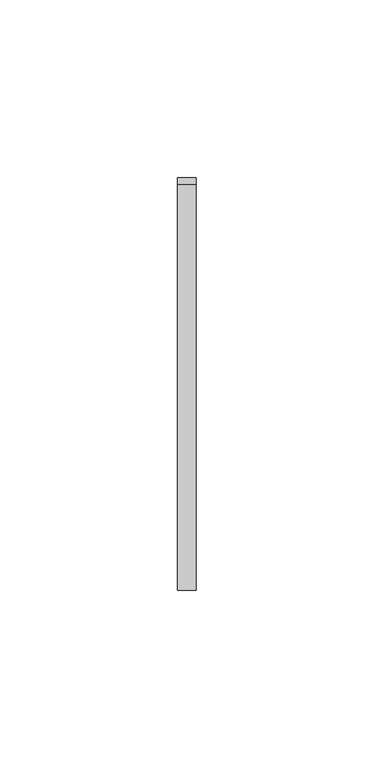
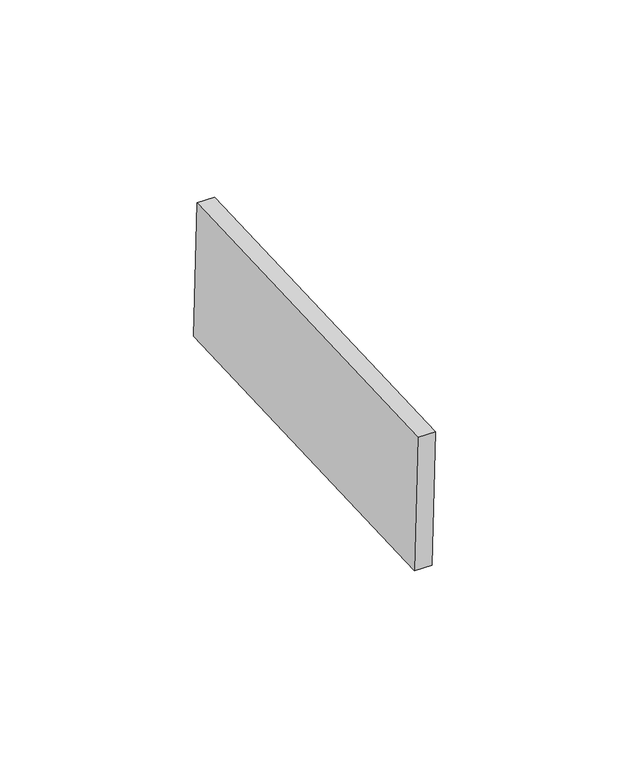
"""IFC4 building model written with IfcOpenShell, lengths in millimetres: proxy geometry, Inner panel:Inner panel:1:Inner panel:1 : Inner panel:Inner panel:300324:2:Inner panel:1:Inner panel:1 : Inner panel:Inner panel:300324:2 : Inner panel:Inner panel:1:Inner panel:1 : Inner panel:Inner panel:300324:300043:83 : Inner panel:Inner panel:1:Inner panel:1 : Inner panel:Inner panel:300324:2:Inner panel:1:Inner panel:1 : Inner panel:Inner panel:300324:2 : Inner panel:Inner panel:1:Inner panel:1 : Inner panel:Inner panel:300324:300043:308120."""

import ifcopenshell
import ifcopenshell.guid

model = None  # the IFC model being written
_history = None  # IfcOwnerHistory: only IFC2X3 demands one
_inside = {}  # id of a spatial element -> (the spatial element, [elements in it])
_under = {}  # id of a project, library or spatial element -> (it, [spatial elements below it])
_declared = {}  # id of a project -> (the project, [libraries it declares])
_typed = {}  # id of a type object -> (the type object, [elements of that type])
_made_of = {}  # id of a material, layer set ... -> (it, [elements and type objects made of it])


def new_model(schema):
    """Start an empty IFC model of exactly this schema.

    Asked for "IFC4X3", IfcOpenShell would pick the latest addendum, in which some entities
    have other attributes; the version numbers below select the first issue.
    IFC2X3 requires an IfcOwnerHistory on every rooted entity: one is made here for all.
    """
    global model, _history
    if schema == "IFC4X3":
        model = ifcopenshell.file(schema_version=(4, 3, 0, 0))
    else:
        model = ifcopenshell.file(schema=schema)
    _inside.clear()
    _under.clear()
    _declared.clear()
    _typed.clear()
    _made_of.clear()
    _history = None
    if model.schema == "IFC2X3":
        org = make("IfcOrganization", Name="unknown")
        user = make(
            "IfcPersonAndOrganization",
            ThePerson=make("IfcPerson", FamilyName="unknown"),
            TheOrganization=org,
        )
        app = make(
            "IfcApplication",
            ApplicationDeveloper=org,
            Version="unknown",
            ApplicationFullName="unknown",
            ApplicationIdentifier="unknown",
        )
        _history = make(
            "IfcOwnerHistory",
            OwningUser=user,
            OwningApplication=app,
            ChangeAction="ADDED",
            CreationDate=0,
        )
    return model


def make(cls, **values):
    """One entity of the class cls with the attributes given. An attribute that is None is left unset."""
    return model.create_entity(
        cls, **{name: value for name, value in values.items() if value is not None}
    )


def rooted(cls, **values):
    """An entity with a GlobalId (a new one), such as an element, a storey or a relation."""
    return make(cls, GlobalId=ifcopenshell.guid.new(), OwnerHistory=_history, **values)


def si_unit(unit_type, name, prefix=None):
    """IfcSIUnit, for example si_unit("LENGTHUNIT", "METRE", prefix="MILLI")."""
    return make("IfcSIUnit", UnitType=unit_type, Prefix=prefix, Name=name)


def assignment(units):
    """IfcUnitAssignment: the units of a project."""
    return None if units is None else make("IfcUnitAssignment", Units=units)


def point(xyz):
    """IfcCartesianPoint."""
    return None if xyz is None else make("IfcCartesianPoint", Coordinates=xyz)


def direction(xyz):
    """IfcDirection."""
    return None if xyz is None else make("IfcDirection", DirectionRatios=xyz)


def frame(location, z_axis=None, x_axis=None):
    """IfcAxis2Placement3D, a coordinate frame: its origin and axes. An axis left out is left unset."""
    return make(
        "IfcAxis2Placement3D",
        Location=point(location),
        Axis=direction(z_axis),
        RefDirection=direction(x_axis),
    )


def origin():
    """The frame at (0, 0, 0) with its axes left unset."""
    return frame((0.0, 0.0, 0.0))


def place(relative_to, where):
    """IfcLocalPlacement: puts the frame where relative to a parent placement (None: the world)."""
    return make(
        "IfcLocalPlacement", PlacementRelTo=relative_to, RelativePlacement=where
    )


def context(
    kind, dimensions, precision=None, world=None, true_north=None, identifier=None
):
    """IfcGeometricRepresentationContext, for example the 3D "Model" context."""
    return make(
        "IfcGeometricRepresentationContext",
        ContextIdentifier=identifier,
        ContextType=kind,
        CoordinateSpaceDimension=dimensions,
        Precision=precision,
        WorldCoordinateSystem=world,
        TrueNorth=true_north,
    )


def project(units=None, contexts=None):
    """IfcProject with its units and contexts."""
    return rooted(
        "IfcProject",
        Name="project",
        RepresentationContexts=contexts,
        UnitsInContext=assignment(units),
    )


def spatial(cls, under=None, at=None, **own):
    """A site, building, storey or space (cls), placed at a placement, below another one or the project."""
    s = rooted(cls, ObjectPlacement=at, **own)
    if under is not None:
        _under.setdefault(under.id(), (under, []))[1].append(s)
    return s


def polyline(points):
    """IfcPolyline through the points."""
    return make("IfcPolyline", Points=[point(p) for p in points])


def outline(outer, holes=None, kind="AREA"):
    """IfcArbitraryClosedProfileDef: a profile drawn as a closed curve; with holes, ...WithVoids."""
    if holes is None:
        return make("IfcArbitraryClosedProfileDef", ProfileType=kind, OuterCurve=outer)
    return make(
        "IfcArbitraryProfileDefWithVoids",
        ProfileType=kind,
        OuterCurve=outer,
        InnerCurves=holes,
    )


def extrude(swept, where, along, depth):
    """IfcExtrudedAreaSolid: the profile swept, set in the frame where, extruded along a direction by depth."""
    return make(
        "IfcExtrudedAreaSolid",
        SweptArea=swept,
        Position=where,
        ExtrudedDirection=direction(along),
        Depth=depth,
    )


def shape(context_of_items, identifier, shape_type, items):
    """IfcShapeRepresentation: the items that make up one representation, for example the "Body"."""
    return make(
        "IfcShapeRepresentation",
        ContextOfItems=context_of_items,
        RepresentationIdentifier=identifier,
        RepresentationType=shape_type,
        Items=items,
    )


def source(mapping_origin, context_of_items, identifier, shape_type, items):
    """IfcRepresentationMap: a shape defined once, which mapped items show again and again."""
    return make(
        "IfcRepresentationMap",
        MappingOrigin=mapping_origin,
        MappedRepresentation=shape(context_of_items, identifier, shape_type, items),
    )


def transform(
    local_origin,
    x_axis=None,
    y_axis=None,
    z_axis=None,
    scale=None,
    scale2=None,
    scale3=None,
    uniform=True,
):
    """IfcCartesianTransformationOperator3D, or its non-uniform kind. x_axis, y_axis, z_axis: its Axis1, 2, 3."""
    if uniform:
        return make(
            "IfcCartesianTransformationOperator3D",
            Axis1=direction(x_axis),
            Axis2=direction(y_axis),
            LocalOrigin=point(local_origin),
            Scale=scale,
            Axis3=direction(z_axis),
        )
    return make(
        "IfcCartesianTransformationOperator3DnonUniform",
        Axis1=direction(x_axis),
        Axis2=direction(y_axis),
        LocalOrigin=point(local_origin),
        Scale=scale,
        Axis3=direction(z_axis),
        Scale2=scale2,
        Scale3=scale3,
    )


def mapped(mapping_source, mapping_target):
    """IfcMappedItem: shows the shape of a source again, moved by a transform."""
    return make(
        "IfcMappedItem", MappingSource=mapping_source, MappingTarget=mapping_target
    )


def made_of(thing, what):
    """Note that an element or type object is made of a material, layer set ...; save() writes the relation."""
    if what is not None:
        _made_of.setdefault(what.id(), (what, []))[1].append(thing)
    return thing


def element(
    cls,
    number,
    at=None,
    inside=None,
    cuts=None,
    type_object=None,
    material=None,
    context=None,
    identifier="Body",
    shape_type=None,
    held_by="IfcProductDefinitionShape",
    body=None,
    shapes=None,
    **own,
):
    """One element of the class cls, such as IfcWall. Its Tag is "e" and its number.

    at: its placement. inside: the storey or other place that contains it. cuts: it is an
    opening in that element (IfcRelVoidsElement). A single representation is given by context,
    identifier, shape_type and body (its items); several are given by shapes. held_by: the class
    of the entity that holds the representations. save() writes the other relations.
    """
    e = rooted(cls, Tag="e%d" % number, ObjectPlacement=at, **own)
    if body is not None:
        shapes = [shape(context, identifier, shape_type, body)]
    if shapes is not None:
        e.Representation = make(held_by, Representations=shapes)
    if inside is not None:
        _inside.setdefault(inside.id(), (inside, []))[1].append(e)
    if cuts is not None:
        rooted(
            "IfcRelVoidsElement", RelatingBuildingElement=cuts, RelatedOpeningElement=e
        )
    if type_object is not None:
        _typed.setdefault(type_object.id(), (type_object, []))[1].append(e)
    return made_of(e, material)


def aggregate(whole, parts):
    """IfcRelAggregates: a whole, such as a stair, and the parts it consists of."""
    return rooted("IfcRelAggregates", RelatingObject=whole, RelatedObjects=parts)


def save(model, path):
    """Write the relations noted so far, then the file.

    IfcRelAggregates (storeys below a building ...), IfcRelContainedInSpatialStructure (elements
    in a storey), IfcRelDefinesByType, IfcRelAssociatesMaterial and IfcRelDeclares: one each for
    every whole, place, type object, material and project.
    """
    for whole, parts in _under.values():
        aggregate(whole, parts)
    for where, things in _inside.values():
        rooted(
            "IfcRelContainedInSpatialStructure",
            RelatedElements=things,
            RelatingStructure=where,
        )
    for kind, things in _typed.values():
        rooted("IfcRelDefinesByType", RelatedObjects=things, RelatingType=kind)
    for what, things in _made_of.values():
        rooted("IfcRelAssociatesMaterial", RelatedObjects=things, RelatingMaterial=what)
    for by, libraries in _declared.values():
        rooted("IfcRelDeclares", RelatingContext=by, RelatedDefinitions=libraries)
    model.write(path)


def generic_models_ed7b09bf(model_context):
    return source(origin(), model_context, "Body", "SweptSolid", [
        extrude(outline(polyline([(0.0, -114.3), (0.0, 0.0), (5.2138089, 0.0), (5.2138089, -114.3), (0.0, -114.3)])), frame((591904.595117, -577458.3096573, 4016.6427799), z_axis=(0.0, -0.04163054471216399, 0.9991330730923527), x_axis=(-1.0, 0.0, 0.0)), (0.0, 0.0, 1.0), 43.2233908),
    ])


if __name__ == "__main__":
    model = new_model("IFC4")
    model_context = context("Model", 3, world=origin())
    ifc_project = project(units=[si_unit("LENGTHUNIT", "METRE", prefix="MILLI")], contexts=[model_context])
    site = spatial("IfcSite", under=ifc_project)
    building = spatial("IfcBuilding", under=site)
    placement = place(None, origin())
    generic_models_shape = generic_models_ed7b09bf(model_context)
    element("IfcBuildingElementProxy", 1, Name="Inner panel:Inner panel:1:Inner panel:1 : Inner panel:Inner panel:300324:2:Inner panel:1:Inner panel:1 : Inner panel:Inner panel:300324:2 : Inner panel:Inner panel:1:Inner panel:1 : Inner panel:Inner panel:300324:300043:83 : Inner panel:Inner panel:1:Inner panel:1 : Inner panel:Inner panel:300324:2:Inner panel:1:Inner panel:1 : Inner panel:Inner panel:300324:2 : Inner panel:Inner panel:1:Inner panel:1 : Inner panel:Inner panel:300324:300043:308120", ObjectType="Inner panel:Inner panel:1:Inner panel:1 : Inner panel:Inner panel:300324:2:Inner panel:1:Inner panel:1 : Inner panel:Inner panel:300324:2 : Inner panel:Inner panel:1:Inner panel:1 : Inner panel:Inner panel:300324:300043:83 : Inner panel:Inner panel:1:Inner panel:1 : Inner panel:Inner panel:300324:2:Inner panel:1:Inner panel:1 : Inner panel:Inner panel:300324:2 : Inner panel:Inner panel:1:Inner panel:1 : Inner panel:Inner panel:300324:300043:308120", at=placement, inside=building, context=model_context, shape_type="MappedRepresentation", body=[
        mapped(generic_models_shape, transform((0.0, 0.0, 0.0), x_axis=(1.0, 0.0, 0.0), y_axis=(0.0, 1.0, 0.0), z_axis=(0.0, 0.0, 1.0))),
    ])
    save(model, "model.ifc")

# Revit data of these elements
# Type "Inner panel:Inner panel:1:Inner panel:1 : Inner panel:Inner panel:300324:2:Inner panel:1:Inner panel:1 : Inner panel:Inner panel:300324:2 : Inner panel:Inner panel:1:Inner panel:1 : Inner panel:Inner panel:300324:300043:83 : Inner panel:Inner panel:1:Inner panel:1 : Inner panel:Inner panel:300324:2:Inner panel:1:Inner panel:1 : Inner panel:Inner panel:300324:2 : Inner panel:Inner panel:1:Inner panel:1 : Inner panel:Inner panel:300324:300043:308120"
#   NameOverride = "Inner panel:Inner panel:1:Inner panel:1 : Inner panel:Inner panel:300324:2:Inner panel:1:Inner panel:1 : Inner panel:Inner panel:300324:2 : Inner panel:Inner panel:1:Inner panel:1 : Inner panel:Inner panel:300324:300043:308120"
#   ObjectTypeOverride = "Inner panel:1:Inner panel:1 : Inner panel:Inner panel:300324:2 : Inner panel:Inner panel:1:Inner panel:1 : Inner panel:Inner panel:300324:300043"
#   Reference = "Inner panel"
#   Tag = "308120"
# Element 1 (IfcBuildingElementProxy, "Inner panel:Inner panel:1:Inner panel:1 : Inner panel:Inner panel:300324:2:Inner panel:1:Inner panel:1 : Inner panel:Inner panel:300324:2 : Inner panel:Inner panel:1:Inner panel:1 : Inner panel:Inner panel:300324:300043:83 : Inner panel:Inner panel:1:Inner panel:1 : Inner panel:Inner panel:300324:2:Inner panel:1:Inner panel:1 : Inner panel:Inner panel:300324:2 : Inner panel:Inner panel:1:Inner panel:1 : Inner panel:Inner panel:300324:300043:308120")
#   Materials on its faces: "SLIDING CLIP"
# Materials
#   "SLIDING CLIP": class "Generic", colour RGB 120 120 120, transparency 0, Cost = 0
